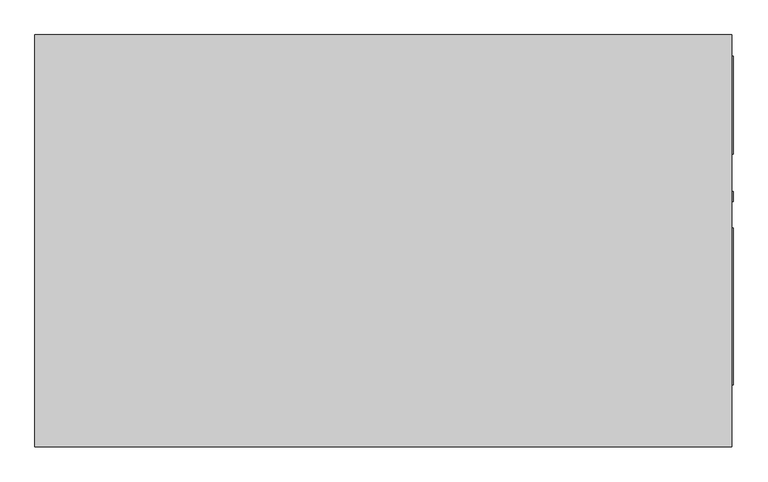
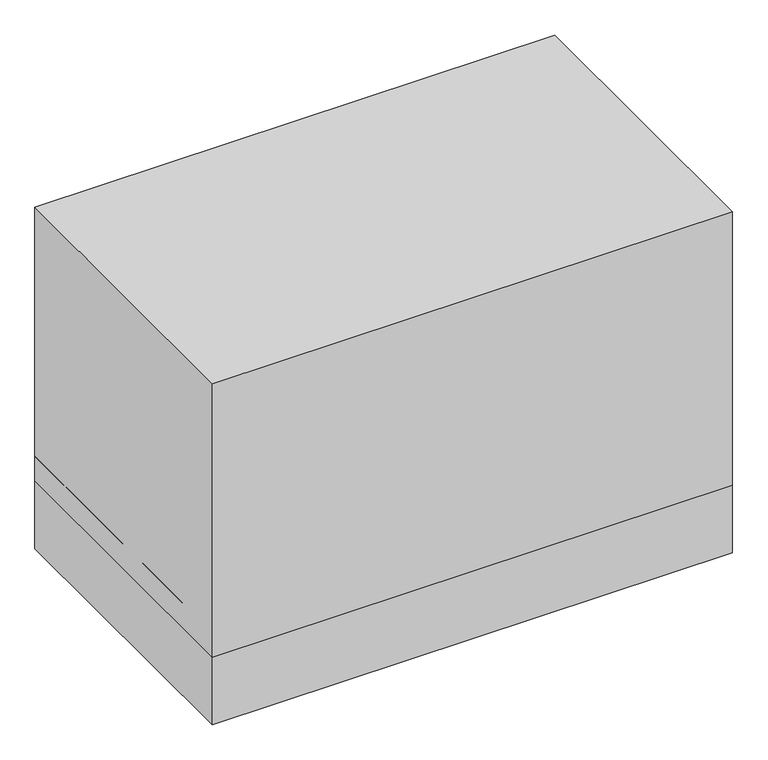
"""IFC4 building model written with IfcOpenShell, lengths in millimetres: proxy geometry, Carrier_48TC_Standard_Efficiency_Gas_Heat_Electric_Cooling_Packaged_Rooftop_Unit_3_to_15_nominal_tons : 6 ton 48TC**07."""

from ifc_helpers import new_model, si_unit, point, frame, frame_2d, origin, origin_with_axes, place, context, project, spatial, polyline, circle_curve, trimmed, segment, composite_curve, outline, extrude, source, transform, mapped, element, save
from ifc_brep_helpers import plane_surface, revolved_surface, advanced_brep


def mechanical_equipment_0a92c70c(model_context):
    return source(origin(), model_context, "Body", "SolidModel", [
        extrude(outline(composite_curve([segment(trimmed(circle_curve(frame_2d((120.65, 438.15)), 13.2953125), [point((107.3546875, 438.15))], [point((133.9453125, 438.15))], False, "CARTESIAN"), True, "CONTINUOUS"), segment(trimmed(circle_curve(frame_2d((120.65, 438.15)), 13.2953125), [point((133.9453125, 438.15))], [point((107.3546875, 438.15))], False, "CARTESIAN"), True, "CONTINUOUS")], self_intersect=False)), frame((944.5625, 0.0, 0.0), z_axis=(1.0, 0.0, 0.0), x_axis=(0.0, 1.0, 0.0)), (0.0, 0.0, 1.0), 3.175),
        advanced_brep(
        [(944.5625, 558.8, 1311.275), (-944.5625, 558.8, 1311.275), (-944.5625, -558.8, 1311.275), (944.5625, -558.8, 1311.275), (944.5625, 558.8, 260.35), (944.5625, -558.8, 260.35), (-944.5625, -558.8, 260.35), (-944.5625, 558.8, 260.35), (858.8375, -400.05, 260.35), (858.8375, 50.8, 260.35), (550.8625, 50.8, 260.35), (550.8625, -400.05, 260.35), (858.8375, 463.55, 260.35), (207.9625, 463.55, 260.35), (207.9625, 187.325, 260.35), (858.8375, 187.325, 260.35), (284.7578125, -88.9, 260.35), (258.1671875, -88.9, 260.35), (-298.45, -247.65, 260.35), (-320.675, -247.65, 260.35), (-295.275, -149.225, 260.35), (-323.85, -149.225, 260.35), (-294.48125, -98.425, 260.35), (-324.64375, -98.425, 260.35), (858.8375, -400.05, 381.0), (550.8625, -400.05, 381.0), (550.8625, 50.8, 381.0), (858.8375, 50.8, 381.0), (858.8375, 463.55, 381.0), (858.8375, 187.325, 381.0), (207.9625, 187.325, 381.0), (207.9625, 463.55, 381.0), (284.7578125, -88.9, 415.925), (258.1671875, -88.9, 415.925), (-298.45, -247.65, 415.925), (-320.675, -247.65, 415.925), (-295.275, -149.225, 415.925), (-323.85, -149.225, 415.925), (-294.48125, -98.425, 415.925), (-324.64375, -98.425, 415.925)],
        [
            (0, 1),
            (1, 2),
            (2, 3),
            (3, 0),
            (4, 5),
            (5, 6),
            (6, 7),
            (7, 4),
            (8, 9),
            (9, 10),
            (10, 11),
            (11, 8),
            (12, 13),
            (13, 14),
            (14, 15),
            (15, 12),
            (16, 17, circle_curve(frame((271.4625, -88.9, 260.35), z_axis=(0.0, 0.0, 1.0), x_axis=(-1.0, 0.0, 0.0)), 13.2953125)),
            (17, 16, circle_curve(frame((271.4625, -88.9, 260.35), z_axis=(0.0, 0.0, 1.0), x_axis=(-1.0, 0.0, 0.0)), 13.2953125)),
            (18, 19, circle_curve(frame((-309.5625, -247.65, 260.35), z_axis=(0.0, 0.0, 1.0), x_axis=(-1.0, 0.0, 0.0)), 11.1125)),
            (19, 18, circle_curve(frame((-309.5625, -247.65, 260.35), z_axis=(0.0, 0.0, 1.0), x_axis=(-1.0, 0.0, 0.0)), 11.1125)),
            (20, 21, circle_curve(frame((-309.5625, -149.225, 260.35), z_axis=(0.0, 0.0, 1.0), x_axis=(-1.0, 0.0, 0.0)), 14.2875)),
            (21, 20, circle_curve(frame((-309.5625, -149.225, 260.35), z_axis=(0.0, 0.0, 1.0), x_axis=(-1.0, 0.0, 0.0)), 14.2875)),
            (22, 23, circle_curve(frame((-309.5625, -98.425, 260.35), z_axis=(0.0, 0.0, 1.0), x_axis=(-1.0, 0.0, 0.0)), 15.08125)),
            (23, 22, circle_curve(frame((-309.5625, -98.425, 260.35), z_axis=(0.0, 0.0, 1.0), x_axis=(-1.0, 0.0, 0.0)), 15.08125)),
            (0, 4),
            (7, 1),
            (6, 2),
            (5, 3),
            (24, 25),
            (25, 26),
            (26, 27),
            (27, 24),
            (27, 9),
            (8, 24),
            (26, 10),
            (25, 11),
            (28, 29),
            (29, 30),
            (30, 31),
            (31, 28),
            (31, 13),
            (12, 28),
            (30, 14),
            (29, 15),
            (32, 33, circle_curve(frame((271.4625, -88.9, 415.925), z_axis=(0.0, 0.0, -1.0), x_axis=(-1.0, 0.0, 0.0)), 13.2953125)),
            (33, 32, circle_curve(frame((271.4625, -88.9, 415.925), z_axis=(0.0, 0.0, -1.0), x_axis=(-1.0, 0.0, 0.0)), 13.2953125)),
            (33, 17),
            (16, 32),
            (34, 35, circle_curve(frame((-309.5625, -247.65, 415.925), z_axis=(0.0, 0.0, -1.0), x_axis=(-1.0, 0.0, 0.0)), 11.1125)),
            (35, 34, circle_curve(frame((-309.5625, -247.65, 415.925), z_axis=(0.0, 0.0, -1.0), x_axis=(-1.0, 0.0, 0.0)), 11.1125)),
            (35, 19),
            (18, 34),
            (36, 37, circle_curve(frame((-309.5625, -149.225, 415.925), z_axis=(0.0, 0.0, -1.0), x_axis=(-1.0, 0.0, 0.0)), 14.2875)),
            (37, 36, circle_curve(frame((-309.5625, -149.225, 415.925), z_axis=(0.0, 0.0, -1.0), x_axis=(-1.0, 0.0, 0.0)), 14.2875)),
            (37, 21),
            (20, 36),
            (38, 39, circle_curve(frame((-309.5625, -98.425, 415.925), z_axis=(0.0, 0.0, -1.0), x_axis=(-1.0, 0.0, 0.0)), 15.08125)),
            (39, 38, circle_curve(frame((-309.5625, -98.425, 415.925), z_axis=(0.0, 0.0, -1.0), x_axis=(-1.0, 0.0, 0.0)), 15.08125)),
            (39, 23),
            (22, 38),
        ],
        [
            plane_surface(frame((-944.5625, 558.8, 1311.275), z_axis=(0.0, 0.0, 1.0), x_axis=(-1.0, 0.0, 0.0))),
            plane_surface(frame((-944.5625, 558.8, 260.35), z_axis=(0.0, 0.0, -1.0), x_axis=(1.0, 0.0, 0.0))),
            plane_surface(frame((944.5625, 558.8, 1311.275), z_axis=(0.0, 1.0, 0.0), x_axis=(0.0, 0.0, -1.0))),
            plane_surface(frame((-944.5625, 558.8, 1311.275), z_axis=(-1.0, 0.0, 0.0), x_axis=(0.0, 0.0, -1.0))),
            plane_surface(frame((-944.5625, -558.8, 1311.275), z_axis=(0.0, -1.0, 0.0), x_axis=(0.0, 0.0, -1.0))),
            plane_surface(frame((944.5625, -558.8, 1311.275), z_axis=(1.0, 0.0, 0.0), x_axis=(0.0, 0.0, -1.0))),
            plane_surface(frame((858.8375, -400.05, 381.0), z_axis=(0.0, 0.0, -1.0), x_axis=(0.0, 1.0, 0.0))),
            plane_surface(frame((858.8375, -400.05, 381.0), z_axis=(-1.0, 0.0, 0.0), x_axis=(0.0, 0.0, -1.0))),
            plane_surface(frame((858.8375, 50.8, 381.0), z_axis=(0.0, -1.0, 0.0), x_axis=(0.0, 0.0, -1.0))),
            plane_surface(frame((550.8625, 50.8, 381.0), z_axis=(1.0, 0.0, 0.0), x_axis=(0.0, 0.0, -1.0))),
            plane_surface(frame((550.8625, -400.05, 381.0), z_axis=(0.0, 1.0, 0.0), x_axis=(0.0, 0.0, -1.0))),
            plane_surface(frame((207.9625, 463.55, 381.0), z_axis=(0.0, 0.0, -1.0), x_axis=(-1.0, 0.0, 0.0))),
            plane_surface(frame((858.8375, 463.55, 381.0), z_axis=(0.0, -1.0, 0.0), x_axis=(0.0, 0.0, -1.0))),
            plane_surface(frame((207.9625, 463.55, 381.0), z_axis=(1.0, 0.0, 0.0), x_axis=(0.0, 0.0, -1.0))),
            plane_surface(frame((207.9625, 187.325, 381.0), z_axis=(0.0, 1.0, 0.0), x_axis=(0.0, 0.0, -1.0))),
            plane_surface(frame((858.8375, 187.325, 381.0), z_axis=(-1.0, 0.0, 0.0), x_axis=(0.0, 0.0, -1.0))),
            plane_surface(frame((258.1671875, -88.9, 415.925), z_axis=(0.0, 0.0, -1.0), x_axis=(0.0, -1.0, 0.0))),
            revolved_surface(polyline([(258.16718749999995, -88.9, 415.925), (258.16718749999995, -88.9, 260.35)]), (271.4625, -88.9, 0.0), (0.0, 0.0, 1.0)),
            plane_surface(frame((-320.675, -247.65, 415.925), z_axis=(0.0, 0.0, -1.0), x_axis=(0.0, -1.0, 0.0))),
            revolved_surface(polyline([(-320.675, -247.65, 415.925), (-320.675, -247.65, 260.35)]), (-309.5625, -247.65, 0.0), (0.0, 0.0, 1.0)),
            plane_surface(frame((-323.85, -149.225, 415.925), z_axis=(0.0, 0.0, -1.0), x_axis=(0.0, -1.0, 0.0))),
            revolved_surface(polyline([(-323.85, -149.225, 415.925), (-323.85, -149.225, 260.35)]), (-309.5625, -149.225, 0.0), (0.0, 0.0, 1.0)),
            plane_surface(frame((-324.64375, -98.425, 415.925), z_axis=(0.0, 0.0, -1.0), x_axis=(0.0, -1.0, 0.0))),
            revolved_surface(polyline([(-324.64375, -98.425, 415.925), (-324.64375, -98.425, 260.35)]), (-309.5625, -98.425, 0.0), (0.0, 0.0, 1.0)),
        ],
        [
            (0, [[1, 2, 3, 4]]),
            (1, [[5, 6, 7, 8], [9, 10, 11, 12], [13, 14, 15, 16], [17, 18], [19, 20], [21, 22], [23, 24]]),
            (2, [[-1, 25, -8, 26]]),
            (3, [[-2, -26, -7, 27]]),
            (4, [[-3, -27, -6, 28]]),
            (5, [[-4, -28, -5, -25]]),
            (6, [[29, 30, 31, 32]]),
            (7, [[-32, 33, -9, 34]]),
            (8, [[-31, 35, -10, -33]]),
            (9, [[-30, 36, -11, -35]]),
            (10, [[-29, -34, -12, -36]]),
            (11, [[37, 38, 39, 40]]),
            (12, [[-40, 41, -13, 42]]),
            (13, [[-39, 43, -14, -41]]),
            (14, [[-38, 44, -15, -43]]),
            (15, [[-37, -42, -16, -44]]),
            (16, [[45, 46]]),
            (17, [[-46, 47, -17, 48]]),
            (17, [[-45, -48, -18, -47]]),
            (18, [[49, 50]]),
            (19, [[-50, 51, -19, 52]]),
            (19, [[-49, -52, -20, -51]]),
            (20, [[53, 54]]),
            (21, [[-54, 55, -21, 56]]),
            (21, [[-53, -56, -22, -55]]),
            (22, [[57, 58]]),
            (23, [[-58, 59, -23, 60]]),
            (23, [[-57, -60, -24, -59]]),
        ],
    ),
        extrude(outline(polyline([(944.5625, 558.8), (944.5625, -558.8), (-944.5625, -558.8), (-944.5625, 558.8), (944.5625, 558.8)]), holes=[polyline([(858.8375, 463.55), (207.9625, 463.55), (207.9625, 187.325), (858.8375, 187.325), (858.8375, 463.55)]), polyline([(858.8375, -400.05), (858.8375, 50.8), (550.8625, 50.8), (550.8625, -400.05), (858.8375, -400.05)]), composite_curve([segment(trimmed(circle_curve(frame_2d((271.4625, -88.9)), 13.2953125), [point((284.7578125, -88.9))], [point((258.1671875, -88.9))], True, "CARTESIAN"), True, "CONTINUOUS"), segment(trimmed(circle_curve(frame_2d((271.4625, -88.9)), 13.2953125), [point((258.1671875, -88.9))], [point((284.7578125, -88.9))], True, "CARTESIAN"), True, "CONTINUOUS")], self_intersect=False), composite_curve([segment(trimmed(circle_curve(frame_2d((-309.5625, -247.65)), 11.1125), [point((-298.45, -247.65))], [point((-320.675, -247.65))], True, "CARTESIAN"), True, "CONTINUOUS"), segment(trimmed(circle_curve(frame_2d((-309.5625, -247.65)), 11.1125), [point((-320.675, -247.65))], [point((-298.45, -247.65))], True, "CARTESIAN"), True, "CONTINUOUS")], self_intersect=False), composite_curve([segment(trimmed(circle_curve(frame_2d((-309.5625, -149.225)), 14.2875), [point((-295.275, -149.225))], [point((-323.85, -149.225))], True, "CARTESIAN"), True, "CONTINUOUS"), segment(trimmed(circle_curve(frame_2d((-309.5625, -149.225)), 14.2875), [point((-323.85, -149.225))], [point((-295.275, -149.225))], True, "CARTESIAN"), True, "CONTINUOUS")], self_intersect=False), composite_curve([segment(trimmed(circle_curve(frame_2d((-309.5625, -98.425)), 15.08125), [point((-294.48125, -98.425))], [point((-324.64375, -98.425))], True, "CARTESIAN"), True, "CONTINUOUS"), segment(trimmed(circle_curve(frame_2d((-309.5625, -98.425)), 15.08125), [point((-324.64375, -98.425))], [point((-294.48125, -98.425))], True, "CARTESIAN"), True, "CONTINUOUS")], self_intersect=False)]), origin_with_axes(), (0.0, 0.0, 1.0), 355.6),
        extrude(outline(polyline([(947.7375, 501.65), (947.7375, 234.95), (944.5625, 234.95), (944.5625, 501.65), (947.7375, 501.65)])), frame((0.0, 0.0, 412.75), z_axis=(0.0, 0.0, 1.0), x_axis=(1.0, 0.0, 0.0)), (0.0, 0.0, 1.0), 638.175),
        extrude(outline(polyline([(947.7375, 34.925), (947.7375, -390.525), (944.5625, -390.525), (944.5625, 34.925), (947.7375, 34.925)])), frame((0.0, 0.0, 415.925), z_axis=(0.0, 0.0, 1.0), x_axis=(1.0, 0.0, 0.0)), (0.0, 0.0, 1.0), 288.925),
    ])


if __name__ == "__main__":
    model = new_model("IFC4")
    model_context = context("Model", 3, world=origin())
    ifc_project = project(units=[si_unit("LENGTHUNIT", "METRE", prefix="MILLI")], contexts=[model_context])
    site = spatial("IfcSite", under=ifc_project)
    building = spatial("IfcBuilding", under=site)
    placement = place(None, origin())
    mechanical_equipment_shape = mechanical_equipment_0a92c70c(model_context)
    element("IfcBuildingElementProxy", 1, Name="Carrier_48TC_Standard_Efficiency_Gas_Heat_Electric_Cooling_Packaged_Rooftop_Unit_3_to_15_nominal_tons : 6 ton 48TC**07", ObjectType="Carrier_48TC_Standard_Efficiency_Gas_Heat_Electric_Cooling_Packaged_Rooftop_Unit_3_to_15_nominal_tons : 6 ton 48TC**07", at=placement, inside=building, context=model_context, shape_type="MappedRepresentation", body=[
        mapped(mechanical_equipment_shape, transform((0.0, 0.0, 0.0), x_axis=(1.0, 0.0, 0.0), y_axis=(0.0, 1.0, 0.0), z_axis=(0.0, 0.0, 1.0))),
    ])
    save(model, "model.ifc")

# Revit data of these elements
# Type "Carrier_48TC_Standard_Efficiency_Gas_Heat_Electric_Cooling_Packaged_Rooftop_Unit_3_to_15_nominal_tons : 6 ton 48TC**07"
#   URL = "www.Carrier.com"
#   Model = "48TC"
#   Manufacturer = "Carrier"
#   Disclaimer = "Manufacturer reserves the right to change, at any time, specifications and designs without notice and without obligation.  Please verify critical parameters with local Carrier commercial sales office."
#   knockout thickness = 0' - 0 1/16"
#   Voltage = 0 V
#   Version = 1
#   TTBY3 = 1' - 0 1/4"
#   TTBY2 = 1' - 4 1/8"
#   TTBY1 = 1' - 6 1/8"
#   TTBX = 2' - 1"
#   TTBPowerR = 0' - 0 9/16"
#   TTBGasR = 0' - 0 19/32"
#   SSSZ = 0' - 6 1/8"
#   SSSY = 0' - 6 5/8"
#   SSSW = 1' - 4 3/4"
#   SSSH = 0' - 11 3/8"
#   SSRZ = 0' - 6"
#   SSRY = 0' - 2 1/4"
#   SSRW = 0' - 10 1/2"
#   SSRH = 2' - 1 1/8"
#   SEER = 0
#   Right clearance = 3' - 0"
#   PWRZ = 1' - 3 3/4"
#   PWRY = 0' - 4 5/8"
#   PWRR = 0' - 1 1/4"
#   ODF2X = 3' - 6"
#   ODF1Y = 1' - 2"
#   ODF1X = 1' - 2"
#   ODF1R = 1' - 1"
#   MOCP = 0 A
#   MCA = 0 A
#   Left clearance = 4' - 0"
#   IEER = 11.2
#   Front clearance = 4' - 0"
#   Fan Z = 4' - 3 5/8"
#   Width = 3' - 8"
#   Length = 6' - 2 3/8"
#   Height = 3' - 5 3/8"
#   EER = 11
#   DSSY = 0' - 6 1/4"
#   DSSX = 0' - 3 3/8"
#   DSSW = 1' - 0 1/8"
#   DSSH = 1' - 5 3/4"
#   DSRY = 0' - 3 3/4"
#   DSRX = 0' - 3 3/8"
#   DSRW = 2' - 1 5/8"
#   DSRH = 0' - 10 7/8"
#   DRNZ = 0' - 7"
#   DRNY = 2' - 2 3/4"
#   DRNR = 0' - 0 67/128"
#   Curb Z = 1' - 2"
#   CFM (nominal) = 0 CFM
#   Back clearance = 3' - 0"
#   Alt Condensate Drain = 0' - 0 67/128"
#   AccypwrR = 0' - 0 7/16"
#   ACY = 1' - 6 1/2"
#   ACX = 2' - 2 1/2"
#   Gas [instance default] = yes
#   Fan 2 on = no
#   Curb_1SLAB_2ROOFCURB_3SNOWCURB = 2
#   Fan 3 on = no
#   Unit material = RTU
#   Curb material = Curb paint
# Element 1 (IfcBuildingElementProxy, "Carrier_48TC_Standard_Efficiency_Gas_Heat_Electric_Cooling_Packaged_Rooftop_Unit_3_to_15_nominal_tons : 6 ton 48TC**07")
#   Materials on its faces: "RTU", "Curb paint", "Mech"
# Materials
#   "RTU": class "Miscellaneous", colour RGB 104 104 104, transparency 0, Cost = 0
#   "Curb paint": class "Miscellaneous", colour RGB 189 187 185, transparency 0
#   "Mech": class "Miscellaneous", colour RGB 235 237 235, transparency 0, Cost = 0
